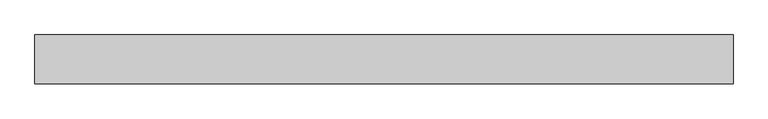
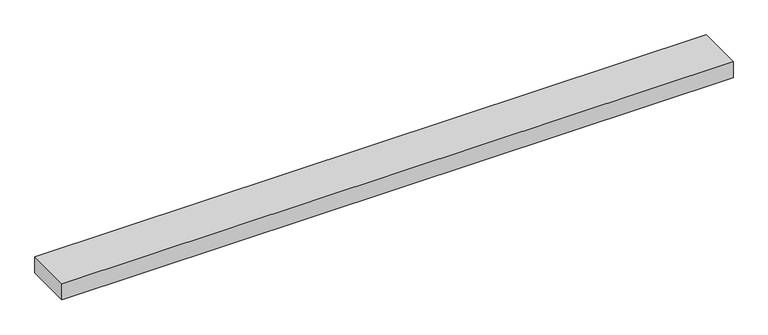
"""IFC4 building model written with IfcOpenShell, lengths in millimetres: proxy geometry, Blocking006 399 : Blocking006 399."""

from ifc_helpers import new_model, si_unit, frame, origin, place, context, project, spatial, polyline, outline, extrude, source, transform, mapped, element, save


def generic_models_2da66233(model_context):
    return source(origin(), model_context, "Body", "SweptSolid", [
        extrude(outline(polyline([(3694.2883192, 9590.6383229), (3694.2883192, 9730.3383229), (5694.2883192, 9730.3383229), (5694.2883192, 9590.6383229), (3694.2883192, 9590.6383229)])), frame((0.0, 0.0, 37445.696), z_axis=(0.0, 0.0, 1.0), x_axis=(1.0, 0.0, 0.0)), (0.0, 0.0, 1.0), 50.8),
    ])


if __name__ == "__main__":
    model = new_model("IFC4")
    model_context = context("Model", 3, world=origin())
    ifc_project = project(units=[si_unit("LENGTHUNIT", "METRE", prefix="MILLI")], contexts=[model_context])
    site = spatial("IfcSite", under=ifc_project)
    building = spatial("IfcBuilding", under=site)
    placement = place(None, origin())
    generic_models_shape = generic_models_2da66233(model_context)
    element("IfcBuildingElementProxy", 1, Name="Blocking006 399 : Blocking006 399", ObjectType="Blocking006 399 : Blocking006 399", at=placement, inside=building, context=model_context, shape_type="MappedRepresentation", body=[
        mapped(generic_models_shape, transform((0.0, 0.0, 0.0), x_axis=(1.0, 0.0, 0.0), y_axis=(0.0, 1.0, 0.0), z_axis=(0.0, 0.0, 1.0))),
    ])
    save(model, "model.ifc")

# Revit data of these elements
# Type "Blocking006 399 : Blocking006 399"
#   NameOverride = "Blocking006"
# Element 1 (IfcBuildingElementProxy, "Blocking006 399 : Blocking006 399")
#   Materials on its faces: "WOOD BLOCKING AS REQUIRED"
# Materials
#   "WOOD BLOCKING AS REQUIRED": class "Unassigned", colour RGB 166 124 85, transparency 0, Cost = 0
